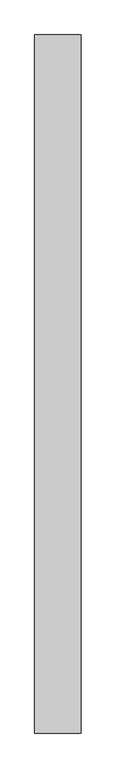
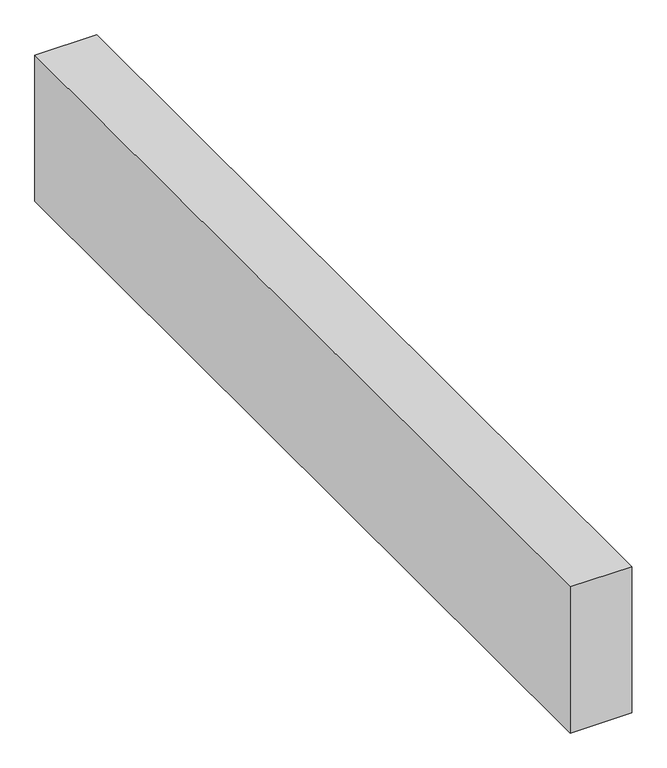
"""IFC4 building model written with IfcOpenShell, lengths in millimetres: proxy geometry, Space Planning Box_hec : Space Planning Box_hec."""

from ifc_helpers import new_model, si_unit, origin, origin_with_axes, place, context, project, spatial, polyline, outline, extrude, source, transform, mapped, element, save


def generic_models_03d31222(model_context):
    return source(origin(), model_context, "Body", "SweptSolid", [
        extrude(outline(polyline([(1200.0, 18000.0), (1200.0, -18000.0), (-1200.0, -18000.0), (-1200.0, 18000.0), (1200.0, 18000.0)])), origin_with_axes(), (0.0, 0.0, 1.0), 6000.0),
    ])


if __name__ == "__main__":
    model = new_model("IFC4")
    model_context = context("Model", 3, world=origin())
    ifc_project = project(units=[si_unit("LENGTHUNIT", "METRE", prefix="MILLI")], contexts=[model_context])
    site = spatial("IfcSite", under=ifc_project)
    building = spatial("IfcBuilding", under=site)
    placement = place(None, origin())
    generic_models_shape = generic_models_03d31222(model_context)
    element("IfcBuildingElementProxy", 1, Name="Space Planning Box_hec : Space Planning Box_hec", ObjectType="Space Planning Box_hec : Space Planning Box_hec", at=placement, inside=building, context=model_context, shape_type="MappedRepresentation", body=[
        mapped(generic_models_shape, transform((0.0, 0.0, 0.0), x_axis=(1.0, 0.0, 0.0), y_axis=(0.0, 1.0, 0.0), z_axis=(0.0, 0.0, 1.0))),
    ])
    save(model, "model.ifc")

# Revit data of these elements
# Type "Space Planning Box_hec : Space Planning Box_hec"
#   Type Comments = "..."
#   Room Name [instance default] = "?"
#   Interior Finish [instance default] = ""
#   Exterior Finish [instance default] = ""
#   Department [instance default] = ""
#   Assembly Code = "..."
#   Width [instance default] = 1524 mm
#   Program Area [instance default] = 0 m²
#   Length [instance default] = 1524 mm
#   Height [instance default] = 1524 mm
#   Area [instance default] = 2.32258 m²
#   Fill Color [instance default] = Cyan
#   Default Elevation = 0
# Element 1 (IfcBuildingElementProxy, "Space Planning Box_hec : Space Planning Box_hec")
#   Room Name = "Corridor"
#   Interior Finish = "IF2-1"
#   Exterior Finish = "EF1"
#   Department = "AR"
#   Width = 2400 mm
#   Program Area = 86.4 m²
#   Length = 36000 mm
#   Height = 6000 mm
#   Area = 86.4 m²
#   Fill Color = Lavender
#   Materials on its faces: "Lavender"
# Materials
#   "Cyan": class "Generic", colour RGB 0 255 255, transparency 0.2, Cost = 0
#   "Lavender": class "Generic", colour RGB 186 85 211, transparency 0.2, Cost = 0
